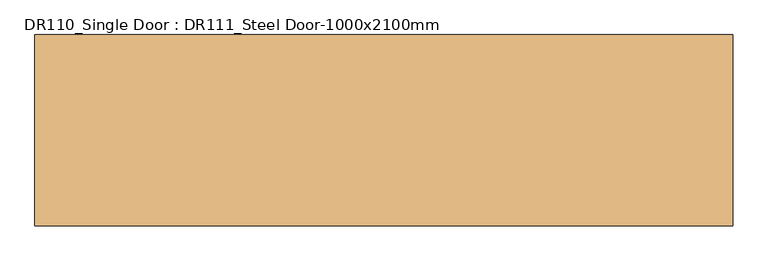
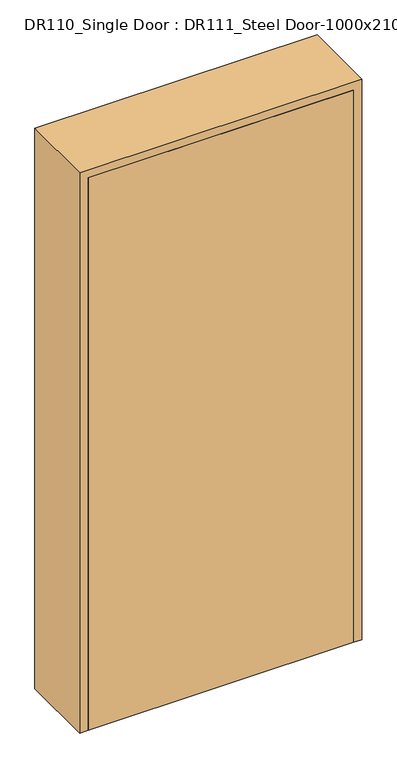
"""IFC4 building model written with IfcOpenShell, lengths in millimetres: door geometry, DR110_Single Door : DR111_Steel Door-1000x2100mm."""

import ifcopenshell
import ifcopenshell.guid

model = None  # the IFC model being written
_history = None  # IfcOwnerHistory: only IFC2X3 demands one
_inside = {}  # id of a spatial element -> (the spatial element, [elements in it])
_under = {}  # id of a project, library or spatial element -> (it, [spatial elements below it])
_declared = {}  # id of a project -> (the project, [libraries it declares])
_typed = {}  # id of a type object -> (the type object, [elements of that type])
_made_of = {}  # id of a material, layer set ... -> (it, [elements and type objects made of it])


def new_model(schema):
    """Start an empty IFC model of exactly this schema.

    Asked for "IFC4X3", IfcOpenShell would pick the latest addendum, in which some entities
    have other attributes; the version numbers below select the first issue.
    IFC2X3 requires an IfcOwnerHistory on every rooted entity: one is made here for all.
    """
    global model, _history
    if schema == "IFC4X3":
        model = ifcopenshell.file(schema_version=(4, 3, 0, 0))
    else:
        model = ifcopenshell.file(schema=schema)
    _inside.clear()
    _under.clear()
    _declared.clear()
    _typed.clear()
    _made_of.clear()
    _history = None
    if model.schema == "IFC2X3":
        org = make("IfcOrganization", Name="unknown")
        user = make(
            "IfcPersonAndOrganization",
            ThePerson=make("IfcPerson", FamilyName="unknown"),
            TheOrganization=org,
        )
        app = make(
            "IfcApplication",
            ApplicationDeveloper=org,
            Version="unknown",
            ApplicationFullName="unknown",
            ApplicationIdentifier="unknown",
        )
        _history = make(
            "IfcOwnerHistory",
            OwningUser=user,
            OwningApplication=app,
            ChangeAction="ADDED",
            CreationDate=0,
        )
    return model


def make(cls, **values):
    """One entity of the class cls with the attributes given. An attribute that is None is left unset."""
    return model.create_entity(
        cls, **{name: value for name, value in values.items() if value is not None}
    )


def rooted(cls, **values):
    """An entity with a GlobalId (a new one), such as an element, a storey or a relation."""
    return make(cls, GlobalId=ifcopenshell.guid.new(), OwnerHistory=_history, **values)


def si_unit(unit_type, name, prefix=None):
    """IfcSIUnit, for example si_unit("LENGTHUNIT", "METRE", prefix="MILLI")."""
    return make("IfcSIUnit", UnitType=unit_type, Prefix=prefix, Name=name)


def assignment(units):
    """IfcUnitAssignment: the units of a project."""
    return None if units is None else make("IfcUnitAssignment", Units=units)


def point(xyz):
    """IfcCartesianPoint."""
    return None if xyz is None else make("IfcCartesianPoint", Coordinates=xyz)


def direction(xyz):
    """IfcDirection."""
    return None if xyz is None else make("IfcDirection", DirectionRatios=xyz)


def frame(location, z_axis=None, x_axis=None):
    """IfcAxis2Placement3D, a coordinate frame: its origin and axes. An axis left out is left unset."""
    return make(
        "IfcAxis2Placement3D",
        Location=point(location),
        Axis=direction(z_axis),
        RefDirection=direction(x_axis),
    )


def origin():
    """The frame at (0, 0, 0) with its axes left unset."""
    return frame((0.0, 0.0, 0.0))


def origin_with_axes():
    """The frame at (0, 0, 0) with the z axis (0, 0, 1) and the x axis (1, 0, 0) written out."""
    return frame((0.0, 0.0, 0.0), z_axis=(0.0, 0.0, 1.0), x_axis=(1.0, 0.0, 0.0))


def place(relative_to, where):
    """IfcLocalPlacement: puts the frame where relative to a parent placement (None: the world)."""
    return make(
        "IfcLocalPlacement", PlacementRelTo=relative_to, RelativePlacement=where
    )


def context(
    kind, dimensions, precision=None, world=None, true_north=None, identifier=None
):
    """IfcGeometricRepresentationContext, for example the 3D "Model" context."""
    return make(
        "IfcGeometricRepresentationContext",
        ContextIdentifier=identifier,
        ContextType=kind,
        CoordinateSpaceDimension=dimensions,
        Precision=precision,
        WorldCoordinateSystem=world,
        TrueNorth=true_north,
    )


def project(units=None, contexts=None):
    """IfcProject with its units and contexts."""
    return rooted(
        "IfcProject",
        Name="project",
        RepresentationContexts=contexts,
        UnitsInContext=assignment(units),
    )


def spatial(cls, under=None, at=None, **own):
    """A site, building, storey or space (cls), placed at a placement, below another one or the project."""
    s = rooted(cls, ObjectPlacement=at, **own)
    if under is not None:
        _under.setdefault(under.id(), (under, []))[1].append(s)
    return s


def polyline(points):
    """IfcPolyline through the points."""
    return make("IfcPolyline", Points=[point(p) for p in points])


def outline(outer, holes=None, kind="AREA"):
    """IfcArbitraryClosedProfileDef: a profile drawn as a closed curve; with holes, ...WithVoids."""
    if holes is None:
        return make("IfcArbitraryClosedProfileDef", ProfileType=kind, OuterCurve=outer)
    return make(
        "IfcArbitraryProfileDefWithVoids",
        ProfileType=kind,
        OuterCurve=outer,
        InnerCurves=holes,
    )


def extrude(swept, where, along, depth):
    """IfcExtrudedAreaSolid: the profile swept, set in the frame where, extruded along a direction by depth."""
    return make(
        "IfcExtrudedAreaSolid",
        SweptArea=swept,
        Position=where,
        ExtrudedDirection=direction(along),
        Depth=depth,
    )


def faces_of(points, faces, orient=None, outer=None):
    """IfcFace entities. A face is a list of loops; a loop is a list of indices into points, from 0.

    orient and outer hold one flag for each loop. By default every Orientation is true, the
    first loop of a face is its IfcFaceOuterBound and the others are IfcFaceBound.
    """
    made = []
    for i, loops in enumerate(faces):
        bounds = []
        for j, loop in enumerate(loops):
            is_outer = j == 0 if outer is None else outer[i][j]
            bounds.append(
                make(
                    "IfcFaceOuterBound" if is_outer else "IfcFaceBound",
                    Bound=make("IfcPolyLoop", Polygon=[points[k] for k in loop]),
                    Orientation=True if orient is None else orient[i][j],
                )
            )
        made.append(make("IfcFace", Bounds=bounds))
    return made


def faceted_brep(points, faces, orient=None, outer=None, voids=None):
    """IfcFacetedBrep: a solid bounded by flat faces; with voids (closed shells), ...WithVoids."""
    shared = [point(p) for p in points]
    hull = make("IfcClosedShell", CfsFaces=faces_of(shared, faces, orient, outer))
    if voids is None:
        return make("IfcFacetedBrep", Outer=hull)
    return make(
        "IfcFacetedBrepWithVoids",
        Outer=hull,
        Voids=[
            make(cls, CfsFaces=faces_of(shared, fs, o, b)) for cls, fs, o, b in voids
        ],
    )


def shape(context_of_items, identifier, shape_type, items):
    """IfcShapeRepresentation: the items that make up one representation, for example the "Body"."""
    return make(
        "IfcShapeRepresentation",
        ContextOfItems=context_of_items,
        RepresentationIdentifier=identifier,
        RepresentationType=shape_type,
        Items=items,
    )


def source(mapping_origin, context_of_items, identifier, shape_type, items):
    """IfcRepresentationMap: a shape defined once, which mapped items show again and again."""
    return make(
        "IfcRepresentationMap",
        MappingOrigin=mapping_origin,
        MappedRepresentation=shape(context_of_items, identifier, shape_type, items),
    )


def transform(
    local_origin,
    x_axis=None,
    y_axis=None,
    z_axis=None,
    scale=None,
    scale2=None,
    scale3=None,
    uniform=True,
):
    """IfcCartesianTransformationOperator3D, or its non-uniform kind. x_axis, y_axis, z_axis: its Axis1, 2, 3."""
    if uniform:
        return make(
            "IfcCartesianTransformationOperator3D",
            Axis1=direction(x_axis),
            Axis2=direction(y_axis),
            LocalOrigin=point(local_origin),
            Scale=scale,
            Axis3=direction(z_axis),
        )
    return make(
        "IfcCartesianTransformationOperator3DnonUniform",
        Axis1=direction(x_axis),
        Axis2=direction(y_axis),
        LocalOrigin=point(local_origin),
        Scale=scale,
        Axis3=direction(z_axis),
        Scale2=scale2,
        Scale3=scale3,
    )


def mapped(mapping_source, mapping_target):
    """IfcMappedItem: shows the shape of a source again, moved by a transform."""
    return make(
        "IfcMappedItem", MappingSource=mapping_source, MappingTarget=mapping_target
    )


def made_of(thing, what):
    """Note that an element or type object is made of a material, layer set ...; save() writes the relation."""
    if what is not None:
        _made_of.setdefault(what.id(), (what, []))[1].append(thing)
    return thing


def element(
    cls,
    number,
    at=None,
    inside=None,
    cuts=None,
    type_object=None,
    material=None,
    context=None,
    identifier="Body",
    shape_type=None,
    held_by="IfcProductDefinitionShape",
    body=None,
    shapes=None,
    **own,
):
    """One element of the class cls, such as IfcWall. Its Tag is "e" and its number.

    at: its placement. inside: the storey or other place that contains it. cuts: it is an
    opening in that element (IfcRelVoidsElement). A single representation is given by context,
    identifier, shape_type and body (its items); several are given by shapes. held_by: the class
    of the entity that holds the representations. save() writes the other relations.
    """
    e = rooted(cls, Tag="e%d" % number, ObjectPlacement=at, **own)
    if body is not None:
        shapes = [shape(context, identifier, shape_type, body)]
    if shapes is not None:
        e.Representation = make(held_by, Representations=shapes)
    if inside is not None:
        _inside.setdefault(inside.id(), (inside, []))[1].append(e)
    if cuts is not None:
        rooted(
            "IfcRelVoidsElement", RelatingBuildingElement=cuts, RelatedOpeningElement=e
        )
    if type_object is not None:
        _typed.setdefault(type_object.id(), (type_object, []))[1].append(e)
    return made_of(e, material)


def aggregate(whole, parts):
    """IfcRelAggregates: a whole, such as a stair, and the parts it consists of."""
    return rooted("IfcRelAggregates", RelatingObject=whole, RelatedObjects=parts)


def save(model, path):
    """Write the relations noted so far, then the file.

    IfcRelAggregates (storeys below a building ...), IfcRelContainedInSpatialStructure (elements
    in a storey), IfcRelDefinesByType, IfcRelAssociatesMaterial and IfcRelDeclares: one each for
    every whole, place, type object, material and project.
    """
    for whole, parts in _under.values():
        aggregate(whole, parts)
    for where, things in _inside.values():
        rooted(
            "IfcRelContainedInSpatialStructure",
            RelatedElements=things,
            RelatingStructure=where,
        )
    for kind, things in _typed.values():
        rooted("IfcRelDefinesByType", RelatedObjects=things, RelatingType=kind)
    for what, things in _made_of.values():
        rooted("IfcRelAssociatesMaterial", RelatedObjects=things, RelatingMaterial=what)
    for by, libraries in _declared.values():
        rooted("IfcRelDeclares", RelatingContext=by, RelatedDefinitions=libraries)
    model.write(path)


def dr110_single_door_dr111_steel_door_1000x2100mm_c730d40a(model_context):
    return source(origin(), model_context, "Body", "SolidModel", [
        extrude(outline(polyline([(470.0, -137.0), (-470.0, -137.0), (-470.0, -102.0), (470.0, -102.0), (470.0, -137.0)])), origin_with_axes(), (0.0, 0.0, 1.0), 2070.0),
        faceted_brep([(470.0, -137.0, 0.0), (470.0, -102.0, 0.0), (450.0, -102.0, 0.0), (450.0, 102.0, 0.0), (470.0, 102.0, 0.0), (470.0, 137.0, 0.0), (500.0, 137.0, 0.0), (500.0, -137.0, 0.0), (500.0, -137.0, 2100.0), (-500.0, -137.0, 2100.0), (-500.0, -137.0, 0.0), (-470.0, -137.0, 0.0), (-470.0, -137.0, 2070.0), (470.0, -137.0, 2070.0), (500.0, 137.0, 2100.0), (470.0, 137.0, 2070.0), (-470.0, 137.0, 2070.0), (-470.0, 137.0, 0.0), (-500.0, 137.0, 0.0), (-500.0, 137.0, 2100.0), (470.0, 102.0, 2070.0), (450.0, 102.0, 2050.0), (-450.0, 102.0, 2050.0), (-450.0, 102.0, 0.0), (-470.0, 102.0, 0.0), (-470.0, 102.0, 2070.0), (450.0, -102.0, 2050.0), (470.0, -102.0, 2070.0), (-470.0, -102.0, 2070.0), (-470.0, -102.0, 0.0), (-450.0, -102.0, 0.0), (-450.0, -102.0, 2050.0)], [[[0, 1, 2, 3, 4, 5, 6, 7]], [[7, 8, 9, 10, 11, 12, 13, 0]], [[6, 14, 8, 7]], [[5, 15, 16, 17, 18, 19, 14, 6]], [[4, 20, 15, 5]], [[3, 21, 22, 23, 24, 25, 20, 4]], [[2, 26, 21, 3]], [[1, 27, 28, 29, 30, 31, 26, 2]], [[0, 13, 27, 1]], [[12, 11, 29, 28]], [[11, 10, 18, 17, 24, 23, 30, 29]], [[19, 18, 10, 9]], [[25, 24, 17, 16]], [[31, 30, 23, 22]], [[14, 19, 9, 8]], [[20, 25, 16, 15]], [[26, 31, 22, 21]], [[13, 12, 28, 27]]]),
    ])


if __name__ == "__main__":
    model = new_model("IFC4")
    model_context = context("Model", 3, world=origin())
    ifc_project = project(units=[si_unit("LENGTHUNIT", "METRE", prefix="MILLI")], contexts=[model_context])
    site = spatial("IfcSite", under=ifc_project)
    building = spatial("IfcBuilding", under=site)
    placement = place(None, origin())
    dr110_single_door_dr111_steel_door_1000x2100mm_shape = dr110_single_door_dr111_steel_door_1000x2100mm_c730d40a(model_context)
    element("IfcDoor", 1, ObjectType="DR110_Single Door : DR111_Steel Door-1000x2100mm", at=placement, inside=building, context=model_context, shape_type="MappedRepresentation", body=[
        mapped(dr110_single_door_dr111_steel_door_1000x2100mm_shape, transform((0.0, 0.0, 0.0), x_axis=(1.0, 0.0, 0.0), y_axis=(0.0, 1.0, 0.0), z_axis=(0.0, 0.0, 1.0))),
    ])
    save(model, "model.ifc")

# Revit data of these elements
# Type "DR110_Single Door : DR111_Steel Door-1000x2100mm"
#   Type Mark = "SD"
#   Analytic Construction = "<None>"
#   프레임 투영 외부. = 25 mm
#   프레임 투영 내부. = 25 mm
#   프레임 폭 = 75 mm
#   Height = 2100 mm
#   Width = 1000 mm
#   Define Thermal Properties by = 1
#   문 패널 = SD1 문 패널
#   문 프레임 = A04AQ098-00002_Steel Door_non FP_single
#   Function = (empty or 0)
#   Wall Closure = (empty or 0)
# Element 1 (IfcDoor, "DR110_Single Door : DR111_Steel Door-1000x2100mm")
#   Materials on its faces: "A04AQ098-00002_Steel Door_non FP_single", "SD1 문 패널"
# Materials
#   "SD1 문 패널": class "금속", colour RGB 247 247 247, transparency 0, Description = "STEEL DOOR (1000Wx2100H)"
#   "A04AQ098-00002_Steel Door_non FP_single": class "금속", colour RGB 247 247 247, transparency 0, Description = "Steel Door", W00) Work Master Code = "A04AQ098-00002", W01) Work Master_Lv1 = "Finishing Work", W02) Work Master_Lv2 = "Door & Window Work", W03) Work Master_Spec.1 = "Steel Door w/ Steel Frame", W04) Work Master_Spec.2 = "Fire Protective Rating: N/A, Single Door", W05) Work Master_Spec.3 = "w/ Hardware & Accessories", Cost = 0
